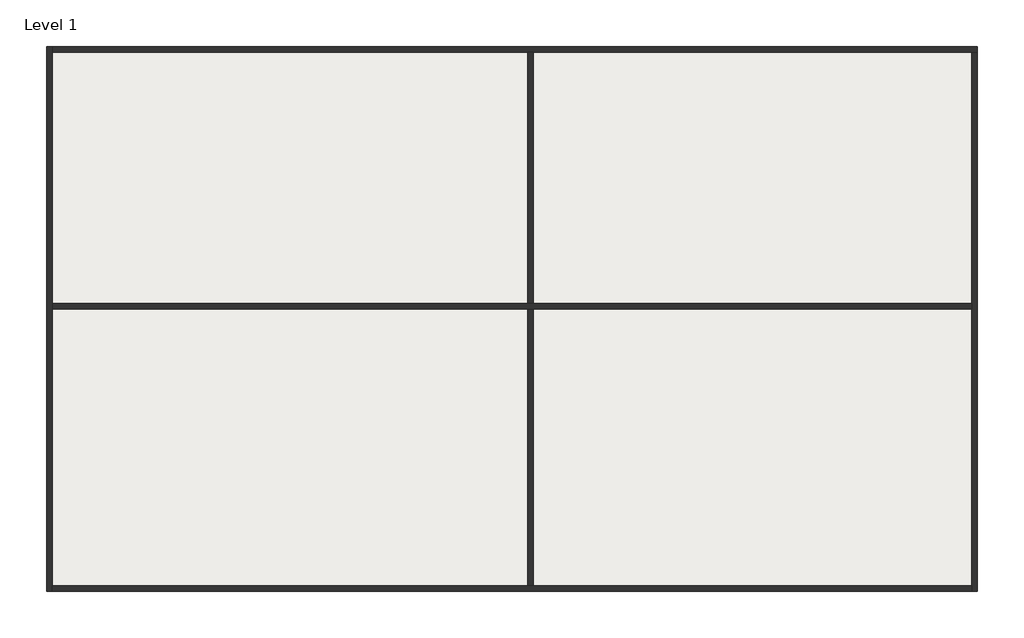
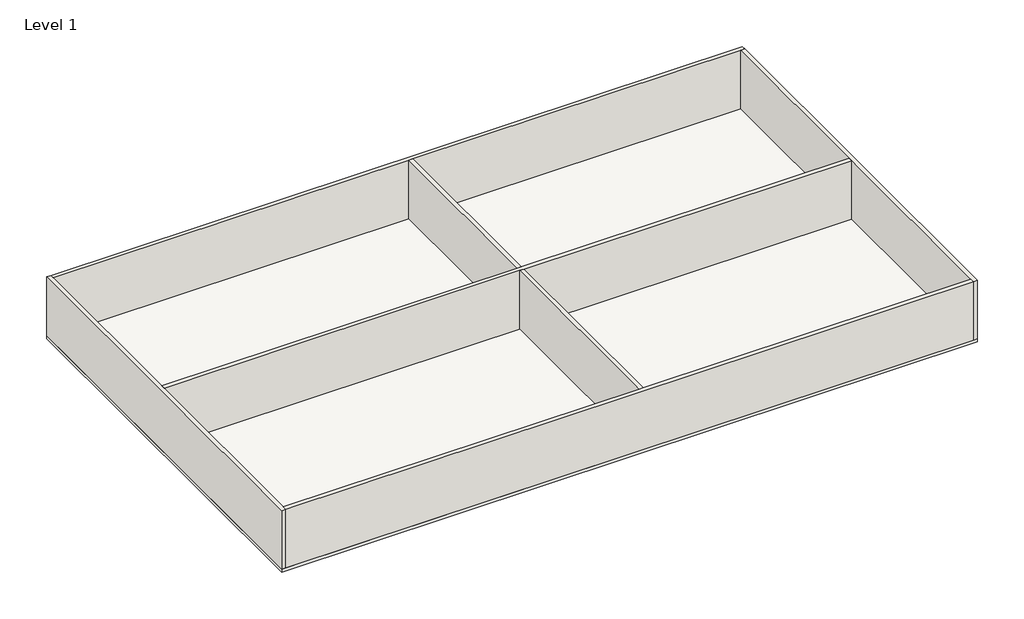
# One storey: 6 walls, 1 slab.
"""IFC4 building model written with IfcOpenShell, lengths in millimetres."""

import ifcopenshell
import ifcopenshell.guid

model = None  # the IFC model being written
_history = None  # IfcOwnerHistory: only IFC2X3 demands one
_inside = {}  # id of a spatial element -> (the spatial element, [elements in it])
_under = {}  # id of a project, library or spatial element -> (it, [spatial elements below it])
_declared = {}  # id of a project -> (the project, [libraries it declares])
_typed = {}  # id of a type object -> (the type object, [elements of that type])
_made_of = {}  # id of a material, layer set ... -> (it, [elements and type objects made of it])


def new_model(schema):
    """Start an empty IFC model of exactly this schema.

    Asked for "IFC4X3", IfcOpenShell would pick the latest addendum, in which some entities
    have other attributes; the version numbers below select the first issue.
    IFC2X3 requires an IfcOwnerHistory on every rooted entity: one is made here for all.
    """
    global model, _history
    if schema == "IFC4X3":
        model = ifcopenshell.file(schema_version=(4, 3, 0, 0))
    else:
        model = ifcopenshell.file(schema=schema)
    _inside.clear()
    _under.clear()
    _declared.clear()
    _typed.clear()
    _made_of.clear()
    _history = None
    if model.schema == "IFC2X3":
        org = make("IfcOrganization", Name="unknown")
        user = make(
            "IfcPersonAndOrganization",
            ThePerson=make("IfcPerson", FamilyName="unknown"),
            TheOrganization=org,
        )
        app = make(
            "IfcApplication",
            ApplicationDeveloper=org,
            Version="unknown",
            ApplicationFullName="unknown",
            ApplicationIdentifier="unknown",
        )
        _history = make(
            "IfcOwnerHistory",
            OwningUser=user,
            OwningApplication=app,
            ChangeAction="ADDED",
            CreationDate=0,
        )
    return model


def make(cls, **values):
    """One entity of the class cls with the attributes given. An attribute that is None is left unset."""
    return model.create_entity(
        cls, **{name: value for name, value in values.items() if value is not None}
    )


def rooted(cls, **values):
    """An entity with a GlobalId (a new one), such as an element, a storey or a relation."""
    return make(cls, GlobalId=ifcopenshell.guid.new(), OwnerHistory=_history, **values)


def si_unit(unit_type, name, prefix=None):
    """IfcSIUnit, for example si_unit("LENGTHUNIT", "METRE", prefix="MILLI")."""
    return make("IfcSIUnit", UnitType=unit_type, Prefix=prefix, Name=name)


def assignment(units):
    """IfcUnitAssignment: the units of a project."""
    return None if units is None else make("IfcUnitAssignment", Units=units)


def point(xyz):
    """IfcCartesianPoint."""
    return None if xyz is None else make("IfcCartesianPoint", Coordinates=xyz)


def direction(xyz):
    """IfcDirection."""
    return None if xyz is None else make("IfcDirection", DirectionRatios=xyz)


def frame(location, z_axis=None, x_axis=None):
    """IfcAxis2Placement3D, a coordinate frame: its origin and axes. An axis left out is left unset."""
    return make(
        "IfcAxis2Placement3D",
        Location=point(location),
        Axis=direction(z_axis),
        RefDirection=direction(x_axis),
    )


def origin():
    """The frame at (0, 0, 0) with its axes left unset."""
    return frame((0.0, 0.0, 0.0))


def origin_with_axes():
    """The frame at (0, 0, 0) with the z axis (0, 0, 1) and the x axis (1, 0, 0) written out."""
    return frame((0.0, 0.0, 0.0), z_axis=(0.0, 0.0, 1.0), x_axis=(1.0, 0.0, 0.0))


def place(relative_to, where):
    """IfcLocalPlacement: puts the frame where relative to a parent placement (None: the world)."""
    return make(
        "IfcLocalPlacement", PlacementRelTo=relative_to, RelativePlacement=where
    )


def context(
    kind, dimensions, precision=None, world=None, true_north=None, identifier=None
):
    """IfcGeometricRepresentationContext, for example the 3D "Model" context."""
    return make(
        "IfcGeometricRepresentationContext",
        ContextIdentifier=identifier,
        ContextType=kind,
        CoordinateSpaceDimension=dimensions,
        Precision=precision,
        WorldCoordinateSystem=world,
        TrueNorth=true_north,
    )


def project(units=None, contexts=None):
    """IfcProject with its units and contexts."""
    return rooted(
        "IfcProject",
        Name="project",
        RepresentationContexts=contexts,
        UnitsInContext=assignment(units),
    )


def spatial(cls, under=None, at=None, **own):
    """A site, building, storey or space (cls), placed at a placement, below another one or the project."""
    s = rooted(cls, ObjectPlacement=at, **own)
    if under is not None:
        _under.setdefault(under.id(), (under, []))[1].append(s)
    return s


def polyline(points):
    """IfcPolyline through the points."""
    return make("IfcPolyline", Points=[point(p) for p in points])


def outline(outer, holes=None, kind="AREA"):
    """IfcArbitraryClosedProfileDef: a profile drawn as a closed curve; with holes, ...WithVoids."""
    if holes is None:
        return make("IfcArbitraryClosedProfileDef", ProfileType=kind, OuterCurve=outer)
    return make(
        "IfcArbitraryProfileDefWithVoids",
        ProfileType=kind,
        OuterCurve=outer,
        InnerCurves=holes,
    )


def extrude(swept, where, along, depth):
    """IfcExtrudedAreaSolid: the profile swept, set in the frame where, extruded along a direction by depth."""
    return make(
        "IfcExtrudedAreaSolid",
        SweptArea=swept,
        Position=where,
        ExtrudedDirection=direction(along),
        Depth=depth,
    )


def faces_of(points, faces, orient=None, outer=None):
    """IfcFace entities. A face is a list of loops; a loop is a list of indices into points, from 0.

    orient and outer hold one flag for each loop. By default every Orientation is true, the
    first loop of a face is its IfcFaceOuterBound and the others are IfcFaceBound.
    """
    made = []
    for i, loops in enumerate(faces):
        bounds = []
        for j, loop in enumerate(loops):
            is_outer = j == 0 if outer is None else outer[i][j]
            bounds.append(
                make(
                    "IfcFaceOuterBound" if is_outer else "IfcFaceBound",
                    Bound=make("IfcPolyLoop", Polygon=[points[k] for k in loop]),
                    Orientation=True if orient is None else orient[i][j],
                )
            )
        made.append(make("IfcFace", Bounds=bounds))
    return made


def faceted_brep(points, faces, orient=None, outer=None, voids=None):
    """IfcFacetedBrep: a solid bounded by flat faces; with voids (closed shells), ...WithVoids."""
    shared = [point(p) for p in points]
    hull = make("IfcClosedShell", CfsFaces=faces_of(shared, faces, orient, outer))
    if voids is None:
        return make("IfcFacetedBrep", Outer=hull)
    return make(
        "IfcFacetedBrepWithVoids",
        Outer=hull,
        Voids=[
            make(cls, CfsFaces=faces_of(shared, fs, o, b)) for cls, fs, o, b in voids
        ],
    )


def shape(context_of_items, identifier, shape_type, items):
    """IfcShapeRepresentation: the items that make up one representation, for example the "Body"."""
    return make(
        "IfcShapeRepresentation",
        ContextOfItems=context_of_items,
        RepresentationIdentifier=identifier,
        RepresentationType=shape_type,
        Items=items,
    )


def made_of(thing, what):
    """Note that an element or type object is made of a material, layer set ...; save() writes the relation."""
    if what is not None:
        _made_of.setdefault(what.id(), (what, []))[1].append(thing)
    return thing


def element(
    cls,
    number,
    at=None,
    inside=None,
    cuts=None,
    type_object=None,
    material=None,
    context=None,
    identifier="Body",
    shape_type=None,
    held_by="IfcProductDefinitionShape",
    body=None,
    shapes=None,
    **own,
):
    """One element of the class cls, such as IfcWall. Its Tag is "e" and its number.

    at: its placement. inside: the storey or other place that contains it. cuts: it is an
    opening in that element (IfcRelVoidsElement). A single representation is given by context,
    identifier, shape_type and body (its items); several are given by shapes. held_by: the class
    of the entity that holds the representations. save() writes the other relations.
    """
    e = rooted(cls, Tag="e%d" % number, ObjectPlacement=at, **own)
    if body is not None:
        shapes = [shape(context, identifier, shape_type, body)]
    if shapes is not None:
        e.Representation = make(held_by, Representations=shapes)
    if inside is not None:
        _inside.setdefault(inside.id(), (inside, []))[1].append(e)
    if cuts is not None:
        rooted(
            "IfcRelVoidsElement", RelatingBuildingElement=cuts, RelatedOpeningElement=e
        )
    if type_object is not None:
        _typed.setdefault(type_object.id(), (type_object, []))[1].append(e)
    return made_of(e, material)


def aggregate(whole, parts):
    """IfcRelAggregates: a whole, such as a stair, and the parts it consists of."""
    return rooted("IfcRelAggregates", RelatingObject=whole, RelatedObjects=parts)


def save(model, path):
    """Write the relations noted so far, then the file.

    IfcRelAggregates (storeys below a building ...), IfcRelContainedInSpatialStructure (elements
    in a storey), IfcRelDefinesByType, IfcRelAssociatesMaterial and IfcRelDeclares: one each for
    every whole, place, type object, material and project.
    """
    for whole, parts in _under.values():
        aggregate(whole, parts)
    for where, things in _inside.values():
        rooted(
            "IfcRelContainedInSpatialStructure",
            RelatedElements=things,
            RelatingStructure=where,
        )
    for kind, things in _typed.values():
        rooted("IfcRelDefinesByType", RelatedObjects=things, RelatingType=kind)
    for what, things in _made_of.values():
        rooted("IfcRelAssociatesMaterial", RelatedObjects=things, RelatingMaterial=what)
    for by, libraries in _declared.values():
        rooted("IfcRelDeclares", RelatingContext=by, RelatedDefinitions=libraries)
    model.write(path)


model = new_model("IFC4")

# Units and contexts
model_context = context("Model", 3, world=origin())
ifc_project = project(units=[si_unit("LENGTHUNIT", "METRE", prefix="MILLI")], contexts=[model_context])

# Site, building, storey
site = spatial("IfcSite", under=ifc_project)
building = spatial("IfcBuilding", under=site)
storey = spatial("IfcBuildingStorey", under=building, Name="Level 1", Elevation=0.0)

# Slab
placement = place(None, origin())
element("IfcSlab", 1, ObjectType="Concrete Slab - 6\"", at=placement, inside=storey, context=model_context, shape_type="SweptSolid", body=[
    extrude(outline(polyline([(-3502.1882593, 10490.08673), (30686.2117407, 10490.08673), (30686.2117407, -9525.11327), (-3502.1882593, -9525.11327), (-3502.1882593, 10490.08673)])), frame((0.0, 0.0, -152.4), z_axis=(0.0, 0.0, 1.0), x_axis=(1.0, 0.0, 0.0)), (0.0, 0.0, 1.0), 152.4),
])

# Walls
element("IfcWall", 2, ObjectType="Generic - 8\"", at=placement, inside=storey, context=model_context, shape_type="Brep", body=[
    faceted_brep([(-3298.9882593, -9525.11327, 0.0), (-3298.9882593, -9321.91327, 0.0), (-3298.9882593, 838.08673, 0.0), (-3298.9882593, 1041.28673, 0.0), (-3298.9882593, 10286.88673, 0.0), (-3298.9882593, 10490.08673, 0.0), (-3298.9882593, 10490.08673, 3048.0), (-3298.9882593, 10286.88673, 3048.0), (-3298.9882593, 1041.28673, 3048.0), (-3298.9882593, 838.08673, 3048.0), (-3298.9882593, -9321.91327, 3048.0), (-3298.9882593, -9525.11327, 3048.0), (-3502.1882593, -9525.11327, 0.0), (-3502.1882593, -9525.11327, 3048.0), (-3502.1882593, 10490.08673, 3048.0), (-3502.1882593, 10490.08673, 0.0)], [[[0, 1, 2, 3, 4, 5, 6, 7, 8, 9, 10, 11]], [[12, 13, 14, 15]], [[5, 4, 3, 2, 1, 0, 12, 15]], [[11, 10, 9, 8, 7, 6, 14, 13]], [[6, 5, 15, 14]], [[0, 11, 13, 12]]]),
])
element("IfcWall", 3, ObjectType="Generic - 8\"", at=placement, inside=storey, context=model_context, shape_type="Brep", body=[
    faceted_brep([(-3298.9882593, 10286.88673, 0.0), (14176.2117407, 10286.88673, 0.0), (14379.4117407, 10286.88673, 0.0), (30483.0117407, 10286.88673, 0.0), (30686.2117407, 10286.88673, 0.0), (30686.2117407, 10286.88673, 3048.0), (30483.0117407, 10286.88673, 3048.0), (14379.4117407, 10286.88673, 3048.0), (14176.2117407, 10286.88673, 3048.0), (-3298.9882593, 10286.88673, 3048.0), (-3298.9882593, 10490.08673, 0.0), (-3298.9882593, 10490.08673, 3048.0), (30686.2117407, 10490.08673, 3048.0), (30686.2117407, 10490.08673, 0.0)], [[[0, 1, 2, 3, 4, 5, 6, 7, 8, 9]], [[10, 11, 12, 13]], [[4, 3, 2, 1, 0, 10, 13]], [[9, 8, 7, 6, 5, 12, 11]], [[0, 9, 11, 10]], [[5, 4, 13, 12]]]),
])
element("IfcWall", 4, ObjectType="Generic - 8\"", at=placement, inside=storey, context=model_context, shape_type="Brep", body=[
    faceted_brep([(30483.0117407, 10286.88673, 0.0), (30483.0117407, 1041.28673, 0.0), (30483.0117407, 838.08673, 0.0), (30483.0117407, -9321.91327, 0.0), (30483.0117407, -9525.11327, 0.0), (30483.0117407, -9525.11327, 3048.0), (30483.0117407, -9321.91327, 3048.0), (30483.0117407, 838.08673, 3048.0), (30483.0117407, 1041.28673, 3048.0), (30483.0117407, 10286.88673, 3048.0), (30686.2117407, 10286.88673, 0.0), (30686.2117407, 10286.88673, 3048.0), (30686.2117407, -9525.11327, 3048.0), (30686.2117407, -9525.11327, 0.0)], [[[0, 1, 2, 3, 4, 5, 6, 7, 8, 9]], [[10, 11, 12, 13]], [[4, 3, 2, 1, 0, 10, 13]], [[9, 8, 7, 6, 5, 12, 11]], [[0, 9, 11, 10]], [[5, 4, 13, 12]]]),
])
element("IfcWall", 5, ObjectType="Generic - 8\"", at=placement, inside=storey, context=model_context, shape_type="Brep", body=[
    faceted_brep([(30483.0117407, -9321.91327, 0.0), (14379.4117407, -9321.91327, 0.0), (14176.2117407, -9321.91327, 0.0), (-3298.9882593, -9321.91327, 0.0), (-3298.9882593, -9321.91327, 3048.0), (14176.2117407, -9321.91327, 3048.0), (14379.4117407, -9321.91327, 3048.0), (30483.0117407, -9321.91327, 3048.0), (30483.0117407, -9525.11327, 0.0), (30483.0117407, -9525.11327, 3048.0), (-3298.9882593, -9525.11327, 3048.0), (-3298.9882593, -9525.11327, 0.0)], [[[0, 1, 2, 3, 4, 5, 6, 7]], [[8, 9, 10, 11]], [[3, 2, 1, 0, 8, 11]], [[7, 6, 5, 4, 10, 9]], [[0, 7, 9, 8]], [[4, 3, 11, 10]]]),
])
element("IfcWall", 6, ObjectType="Generic - 8\"", at=placement, inside=storey, context=model_context, shape_type="Brep", body=[
    faceted_brep([(-3298.9882593, 838.08673, 0.0), (14176.2117407, 838.08673, 0.0), (14379.4117407, 838.08673, 0.0), (30483.0117407, 838.08673, 0.0), (30483.0117407, 838.08673, 3048.0), (14379.4117407, 838.08673, 3048.0), (14176.2117407, 838.08673, 3048.0), (-3298.9882593, 838.08673, 3048.0), (-3298.9882593, 1041.28673, 0.0), (-3298.9882593, 1041.28673, 3048.0), (14176.2117407, 1041.28673, 3048.0), (14379.4117407, 1041.28673, 3048.0), (30483.0117407, 1041.28673, 3048.0), (30483.0117407, 1041.28673, 0.0), (14379.4117407, 1041.28673, 0.0), (14176.2117407, 1041.28673, 0.0)], [[[0, 1, 2, 3, 4, 5, 6, 7]], [[8, 9, 10, 11, 12, 13, 14, 15]], [[3, 2, 1, 0, 8, 15, 14, 13]], [[7, 6, 5, 4, 12, 11, 10, 9]], [[0, 7, 9, 8]], [[4, 3, 13, 12]]]),
])
element("IfcWall", 7, ObjectType="Generic - 8\"", at=placement, inside=storey, context=model_context, shape_type="SweptSolid", body=[
    extrude(outline(polyline([(14176.2117407, 10286.88673), (14379.4117407, 10286.88673), (14379.4117407, 1041.28673), (14176.2117407, 1041.28673), (14176.2117407, 10286.88673)])), origin_with_axes(), (0.0, 0.0, 1.0), 3048.0),
    extrude(outline(polyline([(14379.4117407, -9321.91327), (14176.2117407, -9321.91327), (14176.2117407, 838.08673), (14379.4117407, 838.08673), (14379.4117407, -9321.91327)])), origin_with_axes(), (0.0, 0.0, 1.0), 3048.0),
])

save(model, "model.ifc")

# Revit data of these elements
# Project information
#   Project Issue Date = "Issue Date"
#   Project Status = "Project Status"
#   Client Name = "Owner"
#   Project Address = "Enter address here"
#   Project Name = "Project Name"
#   Project Number = "Project Number"
# Type "Concrete Slab - 6\""
#   Assembly Code = "B1010"
#   Function = 0
#   Layers, outside or top first: 0' - 6" "Concrete, Cast-in-Place gray" (function 1)
# Type "Generic - 8\""
#   Assembly Code = "B2010"
#   Layers, outside or top first: 0' - 8" no material (function 1)
# Element 1 (IfcSlab, "Concrete Slab - 6\"")
#   built-in parameter 1001955 = 1.5708 (stored number, unit not read)
#   Height Offset From Level = 0' - 0"
#   Phase Created = Project Completion
#   Materials on its faces: "Concrete, Cast-in-Place gray"
# Elements 2, 3, 4, 5, 6, 7 (IfcWall, "Generic - 8\"")
#   Top Offset = 0' - 0"
#   Base Offset = 0' - 0"
#   wall height = 10' - 0"
#   Phase Created = Project Completion
#   Base Constraint = Level 1
#   Top Constraint = Level 2
#   Materials on its faces: "Default Wall"
# Materials
#   "Concrete, Cast-in-Place gray": class "Concrete", colour RGB 192 192 192, transparency 0, Description = "Cast-in-place concrete", Cost = 0
#   "Default Wall": class "Miscellaneous", colour RGB 128 128 128, transparency 0, Cost = 0
# Space at (3588.172, 4695.298) mm, phase "Project Completion", upper level "Level 2", upper offset 0' - 0", lower offset 0' - 0"
#   Number = "1"
#   Name = "Space"
#   Actual Lighting Load per area = 0
#   Actual Power Load per area = 0
#   Sensible Heat Gain per person = 378.551 (stored number, unit not read)
#   Specified Lighting Load = 37420.6 (stored number, unit not read)
#   Specified Power Load = 37439.3 (stored number, unit not read)
#   Specified Lighting Load per area = 21.5171 (stored number, unit not read)
#   Specified Power Load per area = 21.5278 (stored number, unit not read)
#   Latent Heat Gain per person = 378.551 (stored number, unit not read)
#   Total Heat Gain per person = 0
#   Area per Person = 25 (stored number, unit not read)
#   Number of People = 69.5644 (stored number, unit not read)
#   Lighting Load Units = 0
#   Power Load Units = 0
#   Return Airflow = 0
#   Occupancy Unit = 1
#   Condition Type = 2
#   Construction Type = none
# Space at (21967.176, 4695.298) mm, phase "Project Completion", upper level "Level 2", upper offset 0' - 0", lower offset 0' - 0"
#   Number = "2"
#   Name = "Space"
#   Actual Lighting Load per area = 0
#   Actual Power Load per area = 0
#   Sensible Heat Gain per person = 0
#   Specified Lighting Load = 15525.3 (stored number, unit not read)
#   Specified Power Load = 9315.2 (stored number, unit not read)
#   Latent Heat Gain per person = 0
#   Total Heat Gain per person = 0
#   Area per Person = 0
#   Number of People = 104.221 (stored number, unit not read)
#   Lighting Load Units = 0
#   Power Load Units = 0
#   Return Airflow = 0
#   Occupancy Unit = -1
#   Condition Type = 2
#   Construction Type = none
# Space at (22075.928, -4602.956) mm, phase "Project Completion", upper level "Level 2", upper offset 0' - 0", lower offset 0' - 0"
#   Number = "3"
#   Name = "Space"
#   Actual Lighting Load per area = 0
#   Actual Power Load per area = 0
#   Sensible Heat Gain per person = 0
#   Specified Lighting Load = 18956.4 (stored number, unit not read)
#   Specified Power Load = 24643.4 (stored number, unit not read)
#   Latent Heat Gain per person = 0
#   Total Heat Gain per person = 0
#   Area per Person = 0
#   Number of People = 5.72644 (stored number, unit not read)
#   Lighting Load Units = 0
#   Power Load Units = 0
#   Return Airflow = 0
#   Occupancy Unit = -1
#   Condition Type = 2
#   Construction Type = none
